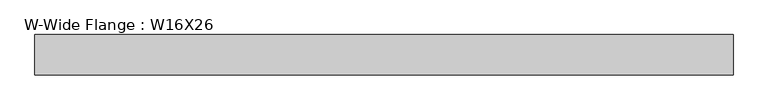
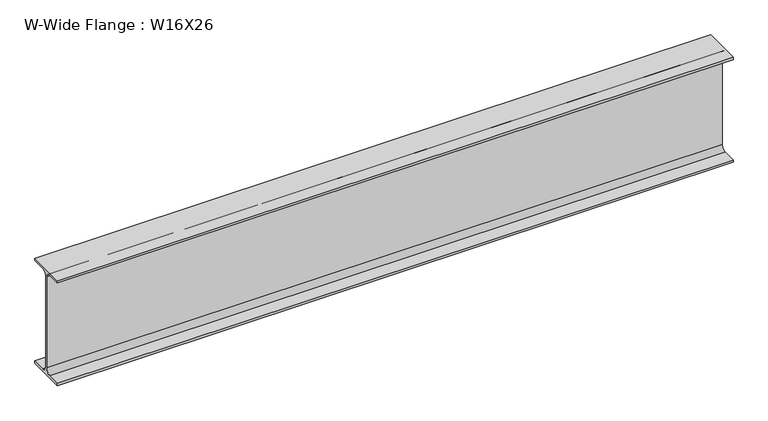
"""IFC4 building model written with IfcOpenShell, lengths in millimetres: beam geometry, W-Wide Flange : W16X26."""

from ifc_helpers import new_model, si_unit, point, frame, frame_2d, origin, place, context, project, spatial, polyline, circle_curve, trimmed, segment, composite_curve, outline, extrude, source, transform, mapped, element, save


def w_wide_flange_w16x26_37e6e801(model_context):
    return source(origin(), model_context, "Body", "SweptSolid", [
        extrude(outline(composite_curve([segment(polyline([(-69.85, -190.5496094), (-21.43125, -190.5496094)]), True, "CONTINUOUS"), segment(trimmed(circle_curve(frame_2d((-21.43125, -172.2933594)), 18.25625), [point((-21.43125, -190.5496094))], [point((-3.175, -172.2933594))], True, "CARTESIAN"), True, "CONTINUOUS"), segment(polyline([(-3.175, -172.2933594), (-3.175, 172.2933594)]), True, "CONTINUOUS"), segment(trimmed(circle_curve(frame_2d((-21.43125, 172.2933594)), 18.25625), [point((-3.175, 172.2933594))], [point((-21.43125, 190.5496094))], True, "CARTESIAN"), True, "CONTINUOUS"), segment(polyline([(-21.43125, 190.5496094), (-69.85, 190.5496094), (-69.85, 199.2808594), (69.85, 199.2808594), (69.85, 190.5496094), (21.43125, 190.5496094)]), True, "CONTINUOUS"), segment(trimmed(circle_curve(frame_2d((21.43125, 172.2933594)), 18.25625), [point((21.43125, 190.5496094))], [point((3.175, 172.2933594))], True, "CARTESIAN"), True, "CONTINUOUS"), segment(polyline([(3.175, 172.2933594), (3.175, -172.2933594)]), True, "CONTINUOUS"), segment(trimmed(circle_curve(frame_2d((21.43125, -172.2933594)), 18.25625), [point((3.175, -172.2933594))], [point((21.43125, -190.5496094))], True, "CARTESIAN"), True, "CONTINUOUS"), segment(polyline([(21.43125, -190.5496094), (69.85, -190.5496094), (69.85, -199.2808594), (-69.85, -199.2808594), (-69.85, -190.5496094)]), True, "CONTINUOUS")], self_intersect=False)), frame((-1079.5, 0.0, 0.0), z_axis=(1.0, 0.0, 0.0), x_axis=(0.0, 1.0, 0.0)), (0.0, 0.0, 1.0), 2423.5884709),
    ])


if __name__ == "__main__":
    model = new_model("IFC4")
    model_context = context("Model", 3, world=origin())
    ifc_project = project(units=[si_unit("LENGTHUNIT", "METRE", prefix="MILLI")], contexts=[model_context])
    site = spatial("IfcSite", under=ifc_project)
    building = spatial("IfcBuilding", under=site)
    placement = place(None, origin())
    w_wide_flange_w16x26_shape = w_wide_flange_w16x26_37e6e801(model_context)
    element("IfcBeam", 1, ObjectType="W-Wide Flange : W16X26", at=placement, inside=building, context=model_context, shape_type="MappedRepresentation", body=[
        mapped(w_wide_flange_w16x26_shape, transform((0.0, 0.0, 0.0), x_axis=(1.0, 0.0, 0.0), y_axis=(0.0, 1.0, 0.0), z_axis=(0.0, 0.0, 1.0))),
    ])
    save(model, "model.ifc")

# Revit data of these elements
# Type "W-Wide Flange : W16X26"
#   Assembly Code = "B10"
#   W = 26
#   Start Extension Calculation [instance default] = 10' - 0"
#   Start Extension [instance default] = -0' - 0 1/2"
#   End Extension Calculation [instance default] = 10' - 0"
#   End Extension [instance default] = -0' - 0 1/2"
#   Length [instance default] = 5' - 0"
#   bf = 0' - 5 1/2"
#   d = 1' - 3 177/256"
#   k = 0' - 1 1/16"
#   k2 = 0' - 0 23/32"
#   tf = 0' - 0 11/32"
#   tw = 0' - 0 1/4"
#   A = 0.05 SF
#   Beam Material [instance default] = Metal - Steel - ASTM A992
# Element 1 (IfcBeam, "W-Wide Flange : W16X26")
#   End Extension Calculation = 10' - 8.66101"
#   End Extension = 0' - 8.16101"
#   Materials on its faces: "Metal - Steel - ASTM A992"
# Materials
#   "Metal - Steel - ASTM A992": class "Metal", colour RGB 128 0 0, transparency 0
